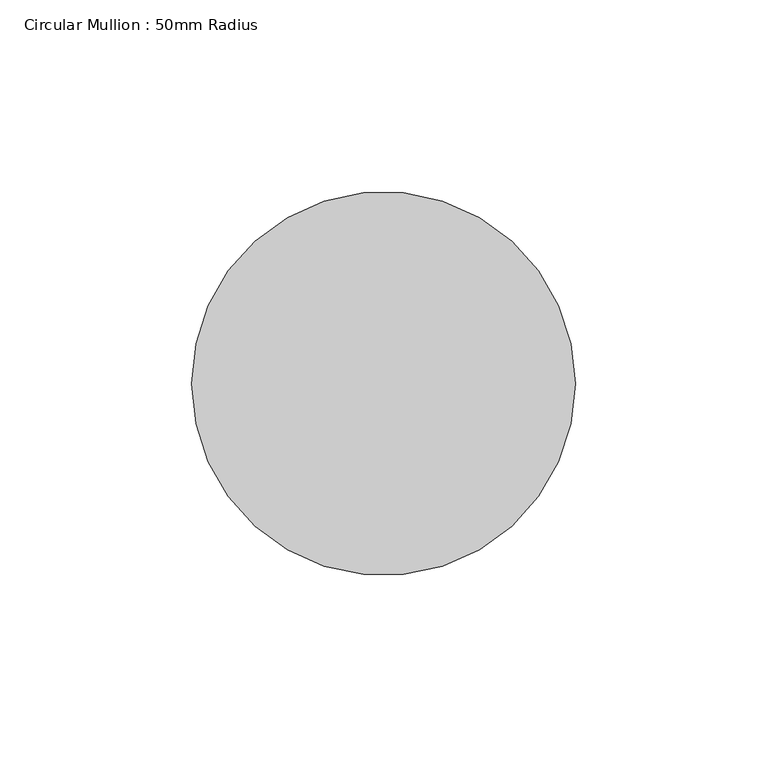
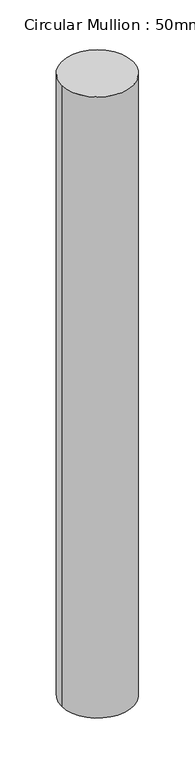
"""IFC4 building model written with IfcOpenShell, lengths in millimetres: member geometry, Circular Mullion : 50mm Radius."""

from ifc_helpers import new_model, si_unit, point, frame, origin, origin_2d, place, context, project, spatial, circle_curve, trimmed, segment, composite_curve, outline, extrude, source, transform, mapped, element, save


def circular_mullion_50mm_radius_8e720566(model_context):
    return source(origin(), model_context, "Body", "SweptSolid", [
        extrude(outline(composite_curve([segment(trimmed(circle_curve(origin_2d(), 50.0), [point((50.0, 0.0))], [point((-50.0, 0.0))], False, "CARTESIAN"), True, "CONTINUOUS"), segment(trimmed(circle_curve(origin_2d(), 50.0), [point((-50.0, 0.0))], [point((50.0, 0.0))], False, "CARTESIAN"), True, "CONTINUOUS")], self_intersect=False)), frame((0.0, 0.0, -921.037419), z_axis=(0.0, 0.0, 1.0), x_axis=(1.0, 0.0, 0.0)), (0.0, 0.0, 1.0), 921.037419),
    ])


if __name__ == "__main__":
    model = new_model("IFC4")
    model_context = context("Model", 3, world=origin())
    ifc_project = project(units=[si_unit("LENGTHUNIT", "METRE", prefix="MILLI")], contexts=[model_context])
    site = spatial("IfcSite", under=ifc_project)
    building = spatial("IfcBuilding", under=site)
    placement = place(None, origin())
    circular_mullion_50mm_radius_shape = circular_mullion_50mm_radius_8e720566(model_context)
    element("IfcMember", 1, ObjectType="Circular Mullion : 50mm Radius", at=placement, inside=building, context=model_context, shape_type="MappedRepresentation", body=[
        mapped(circular_mullion_50mm_radius_shape, transform((0.0, 0.0, 0.0), x_axis=(1.0, 0.0, 0.0), y_axis=(0.0, 1.0, 0.0), z_axis=(0.0, 0.0, 1.0))),
    ])
    save(model, "model.ifc")

# Revit data of these elements
# Type "Circular Mullion : 50mm Radius"
#   built-in parameter 1007350 = 0.164042 (stored number, unit not read)
# Element 1 (IfcMember, "Circular Mullion : 50mm Radius")
#   Materials on its faces: "Aluminium"
# Materials
#   "Aluminium": class "Metal", colour RGB 247 247 247, transparency 0, Description = "Aluminium 6061", Cost = 0
